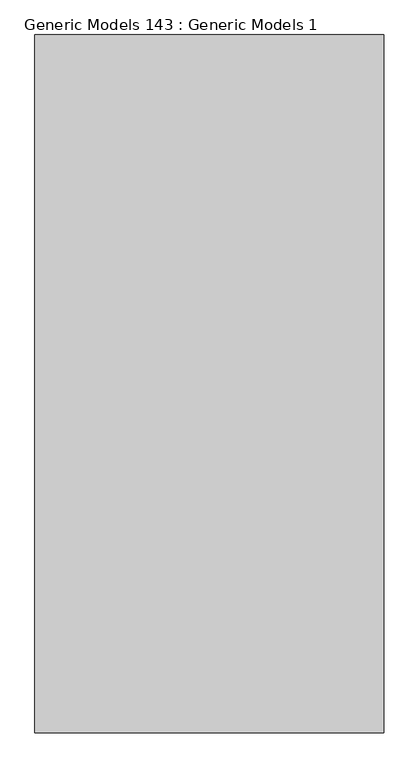
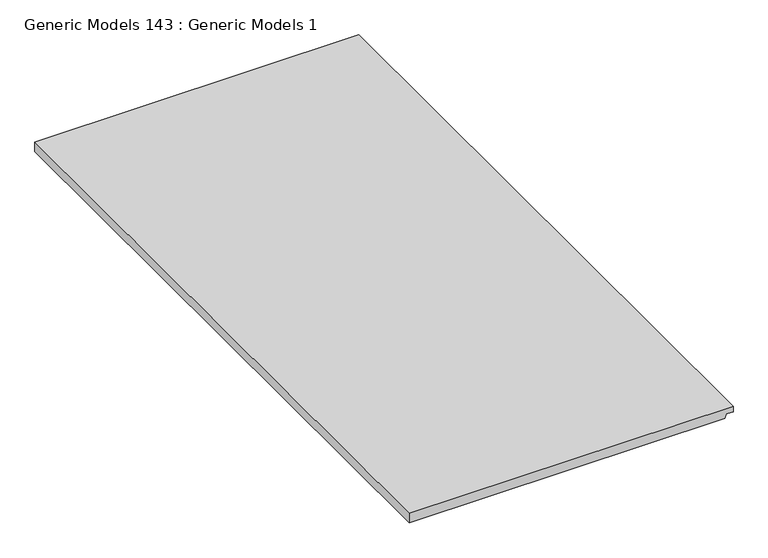
"""IFC4 building model written with IfcOpenShell, lengths in millimetres: proxy geometry, Generic Models 143 : Generic Models 1."""

import ifcopenshell
import ifcopenshell.guid

model = None  # the IFC model being written
_history = None  # IfcOwnerHistory: only IFC2X3 demands one
_inside = {}  # id of a spatial element -> (the spatial element, [elements in it])
_under = {}  # id of a project, library or spatial element -> (it, [spatial elements below it])
_declared = {}  # id of a project -> (the project, [libraries it declares])
_typed = {}  # id of a type object -> (the type object, [elements of that type])
_made_of = {}  # id of a material, layer set ... -> (it, [elements and type objects made of it])


def new_model(schema):
    """Start an empty IFC model of exactly this schema.

    Asked for "IFC4X3", IfcOpenShell would pick the latest addendum, in which some entities
    have other attributes; the version numbers below select the first issue.
    IFC2X3 requires an IfcOwnerHistory on every rooted entity: one is made here for all.
    """
    global model, _history
    if schema == "IFC4X3":
        model = ifcopenshell.file(schema_version=(4, 3, 0, 0))
    else:
        model = ifcopenshell.file(schema=schema)
    _inside.clear()
    _under.clear()
    _declared.clear()
    _typed.clear()
    _made_of.clear()
    _history = None
    if model.schema == "IFC2X3":
        org = make("IfcOrganization", Name="unknown")
        user = make(
            "IfcPersonAndOrganization",
            ThePerson=make("IfcPerson", FamilyName="unknown"),
            TheOrganization=org,
        )
        app = make(
            "IfcApplication",
            ApplicationDeveloper=org,
            Version="unknown",
            ApplicationFullName="unknown",
            ApplicationIdentifier="unknown",
        )
        _history = make(
            "IfcOwnerHistory",
            OwningUser=user,
            OwningApplication=app,
            ChangeAction="ADDED",
            CreationDate=0,
        )
    return model


def make(cls, **values):
    """One entity of the class cls with the attributes given. An attribute that is None is left unset."""
    return model.create_entity(
        cls, **{name: value for name, value in values.items() if value is not None}
    )


def rooted(cls, **values):
    """An entity with a GlobalId (a new one), such as an element, a storey or a relation."""
    return make(cls, GlobalId=ifcopenshell.guid.new(), OwnerHistory=_history, **values)


def si_unit(unit_type, name, prefix=None):
    """IfcSIUnit, for example si_unit("LENGTHUNIT", "METRE", prefix="MILLI")."""
    return make("IfcSIUnit", UnitType=unit_type, Prefix=prefix, Name=name)


def assignment(units):
    """IfcUnitAssignment: the units of a project."""
    return None if units is None else make("IfcUnitAssignment", Units=units)


def point(xyz):
    """IfcCartesianPoint."""
    return None if xyz is None else make("IfcCartesianPoint", Coordinates=xyz)


def direction(xyz):
    """IfcDirection."""
    return None if xyz is None else make("IfcDirection", DirectionRatios=xyz)


def frame(location, z_axis=None, x_axis=None):
    """IfcAxis2Placement3D, a coordinate frame: its origin and axes. An axis left out is left unset."""
    return make(
        "IfcAxis2Placement3D",
        Location=point(location),
        Axis=direction(z_axis),
        RefDirection=direction(x_axis),
    )


def origin():
    """The frame at (0, 0, 0) with its axes left unset."""
    return frame((0.0, 0.0, 0.0))


def place(relative_to, where):
    """IfcLocalPlacement: puts the frame where relative to a parent placement (None: the world)."""
    return make(
        "IfcLocalPlacement", PlacementRelTo=relative_to, RelativePlacement=where
    )


def context(
    kind, dimensions, precision=None, world=None, true_north=None, identifier=None
):
    """IfcGeometricRepresentationContext, for example the 3D "Model" context."""
    return make(
        "IfcGeometricRepresentationContext",
        ContextIdentifier=identifier,
        ContextType=kind,
        CoordinateSpaceDimension=dimensions,
        Precision=precision,
        WorldCoordinateSystem=world,
        TrueNorth=true_north,
    )


def project(units=None, contexts=None):
    """IfcProject with its units and contexts."""
    return rooted(
        "IfcProject",
        Name="project",
        RepresentationContexts=contexts,
        UnitsInContext=assignment(units),
    )


def spatial(cls, under=None, at=None, **own):
    """A site, building, storey or space (cls), placed at a placement, below another one or the project."""
    s = rooted(cls, ObjectPlacement=at, **own)
    if under is not None:
        _under.setdefault(under.id(), (under, []))[1].append(s)
    return s


def polyline(points):
    """IfcPolyline through the points."""
    return make("IfcPolyline", Points=[point(p) for p in points])


def outline(outer, holes=None, kind="AREA"):
    """IfcArbitraryClosedProfileDef: a profile drawn as a closed curve; with holes, ...WithVoids."""
    if holes is None:
        return make("IfcArbitraryClosedProfileDef", ProfileType=kind, OuterCurve=outer)
    return make(
        "IfcArbitraryProfileDefWithVoids",
        ProfileType=kind,
        OuterCurve=outer,
        InnerCurves=holes,
    )


def extrude(swept, where, along, depth):
    """IfcExtrudedAreaSolid: the profile swept, set in the frame where, extruded along a direction by depth."""
    return make(
        "IfcExtrudedAreaSolid",
        SweptArea=swept,
        Position=where,
        ExtrudedDirection=direction(along),
        Depth=depth,
    )


def shape(context_of_items, identifier, shape_type, items):
    """IfcShapeRepresentation: the items that make up one representation, for example the "Body"."""
    return make(
        "IfcShapeRepresentation",
        ContextOfItems=context_of_items,
        RepresentationIdentifier=identifier,
        RepresentationType=shape_type,
        Items=items,
    )


def source(mapping_origin, context_of_items, identifier, shape_type, items):
    """IfcRepresentationMap: a shape defined once, which mapped items show again and again."""
    return make(
        "IfcRepresentationMap",
        MappingOrigin=mapping_origin,
        MappedRepresentation=shape(context_of_items, identifier, shape_type, items),
    )


def transform(
    local_origin,
    x_axis=None,
    y_axis=None,
    z_axis=None,
    scale=None,
    scale2=None,
    scale3=None,
    uniform=True,
):
    """IfcCartesianTransformationOperator3D, or its non-uniform kind. x_axis, y_axis, z_axis: its Axis1, 2, 3."""
    if uniform:
        return make(
            "IfcCartesianTransformationOperator3D",
            Axis1=direction(x_axis),
            Axis2=direction(y_axis),
            LocalOrigin=point(local_origin),
            Scale=scale,
            Axis3=direction(z_axis),
        )
    return make(
        "IfcCartesianTransformationOperator3DnonUniform",
        Axis1=direction(x_axis),
        Axis2=direction(y_axis),
        LocalOrigin=point(local_origin),
        Scale=scale,
        Axis3=direction(z_axis),
        Scale2=scale2,
        Scale3=scale3,
    )


def mapped(mapping_source, mapping_target):
    """IfcMappedItem: shows the shape of a source again, moved by a transform."""
    return make(
        "IfcMappedItem", MappingSource=mapping_source, MappingTarget=mapping_target
    )


def made_of(thing, what):
    """Note that an element or type object is made of a material, layer set ...; save() writes the relation."""
    if what is not None:
        _made_of.setdefault(what.id(), (what, []))[1].append(thing)
    return thing


def element(
    cls,
    number,
    at=None,
    inside=None,
    cuts=None,
    type_object=None,
    material=None,
    context=None,
    identifier="Body",
    shape_type=None,
    held_by="IfcProductDefinitionShape",
    body=None,
    shapes=None,
    **own,
):
    """One element of the class cls, such as IfcWall. Its Tag is "e" and its number.

    at: its placement. inside: the storey or other place that contains it. cuts: it is an
    opening in that element (IfcRelVoidsElement). A single representation is given by context,
    identifier, shape_type and body (its items); several are given by shapes. held_by: the class
    of the entity that holds the representations. save() writes the other relations.
    """
    e = rooted(cls, Tag="e%d" % number, ObjectPlacement=at, **own)
    if body is not None:
        shapes = [shape(context, identifier, shape_type, body)]
    if shapes is not None:
        e.Representation = make(held_by, Representations=shapes)
    if inside is not None:
        _inside.setdefault(inside.id(), (inside, []))[1].append(e)
    if cuts is not None:
        rooted(
            "IfcRelVoidsElement", RelatingBuildingElement=cuts, RelatedOpeningElement=e
        )
    if type_object is not None:
        _typed.setdefault(type_object.id(), (type_object, []))[1].append(e)
    return made_of(e, material)


def aggregate(whole, parts):
    """IfcRelAggregates: a whole, such as a stair, and the parts it consists of."""
    return rooted("IfcRelAggregates", RelatingObject=whole, RelatedObjects=parts)


def save(model, path):
    """Write the relations noted so far, then the file.

    IfcRelAggregates (storeys below a building ...), IfcRelContainedInSpatialStructure (elements
    in a storey), IfcRelDefinesByType, IfcRelAssociatesMaterial and IfcRelDeclares: one each for
    every whole, place, type object, material and project.
    """
    for whole, parts in _under.values():
        aggregate(whole, parts)
    for where, things in _inside.values():
        rooted(
            "IfcRelContainedInSpatialStructure",
            RelatedElements=things,
            RelatingStructure=where,
        )
    for kind, things in _typed.values():
        rooted("IfcRelDefinesByType", RelatedObjects=things, RelatingType=kind)
    for what, things in _made_of.values():
        rooted("IfcRelAssociatesMaterial", RelatedObjects=things, RelatingMaterial=what)
    for by, libraries in _declared.values():
        rooted("IfcRelDeclares", RelatingContext=by, RelatedDefinitions=libraries)
    model.write(path)


def generic_models_143_generic_models_1_02ed30d2(model_context):
    return source(origin(), model_context, "Body", "SweptSolid", [
        extrude(outline(polyline([(2027.354361, 46814.4534123), (2027.354361, 46204.8534123), (2008.304361, 46204.8534123), (2008.304361, 46798.8643986), (2016.241861, 46801.7534123), (2016.241861, 46814.4534123), (2027.354361, 46814.4534123)])), frame((0.0, 0.0, 0.0), z_axis=(0.0, 1.0, 0.0), x_axis=(0.0, 0.0, 1.0)), (0.0, 0.0, 1.0), 1219.2),
    ])


if __name__ == "__main__":
    model = new_model("IFC4")
    model_context = context("Model", 3, world=origin())
    ifc_project = project(units=[si_unit("LENGTHUNIT", "METRE", prefix="MILLI")], contexts=[model_context])
    site = spatial("IfcSite", under=ifc_project)
    building = spatial("IfcBuilding", under=site)
    placement = place(None, origin())
    generic_models_143_generic_models_1_shape = generic_models_143_generic_models_1_02ed30d2(model_context)
    element("IfcBuildingElementProxy", 1, Name="Generic Models 143 : Generic Models 1", ObjectType="Generic Models 143 : Generic Models 1", at=placement, inside=building, context=model_context, shape_type="MappedRepresentation", body=[
        mapped(generic_models_143_generic_models_1_shape, transform((0.0, 0.0, 0.0), x_axis=(1.0, 0.0, 0.0), y_axis=(0.0, 1.0, 0.0), z_axis=(0.0, 0.0, 1.0))),
    ])
    save(model, "model.ifc")

# Revit data of these elements
# Element 1 (IfcBuildingElementProxy, "Generic Models 143 : Generic Models 1")
#   Materials on its faces: "CEILING AS SCHEDULED"
# Materials
#   "CEILING AS SCHEDULED": class "Generic", colour RGB 255 255 255, transparency 0, Cost = 0
